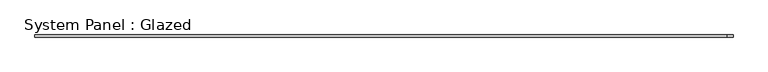
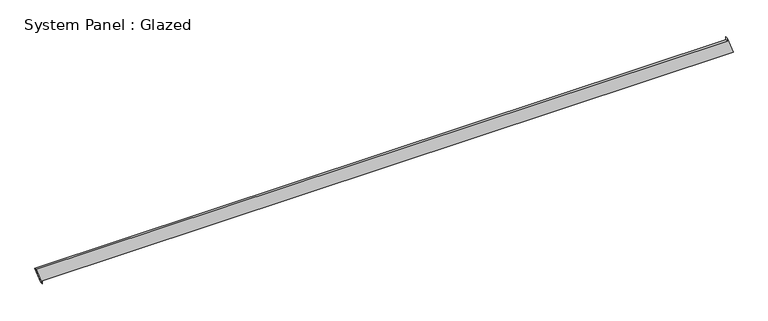
"""IFC4 building model written with IfcOpenShell, lengths in millimetres: plate geometry, System Panel : Glazed."""

from ifc_helpers import new_model, si_unit, frame, origin, place, context, project, spatial, polyline, outline, extrude, source, transform, mapped, element, save


def system_panel_glazed_d03e2e0c(model_context):
    return source(origin(), model_context, "Body", "SweptSolid", [
        extrude(outline(polyline([(0.0, -3959.0543609), (35.3553391, -3959.0543609), (35.3553391, 4027.7767133), (234.8330521, 3959.2965957), (199.477713, 3959.2970385), (199.3776864, -4027.7767133), (0.0, -3959.0543609)])), frame((0.0, -49.5, 0.0), z_axis=(0.0, 1.0, 0.0), x_axis=(0.0, 0.0, 1.0)), (0.0, 0.0, 1.0), 25.0),
    ])


if __name__ == "__main__":
    model = new_model("IFC4")
    model_context = context("Model", 3, world=origin())
    ifc_project = project(units=[si_unit("LENGTHUNIT", "METRE", prefix="MILLI")], contexts=[model_context])
    site = spatial("IfcSite", under=ifc_project)
    building = spatial("IfcBuilding", under=site)
    placement = place(None, origin())
    system_panel_glazed_shape = system_panel_glazed_d03e2e0c(model_context)
    element("IfcPlate", 1, ObjectType="System Panel : Glazed", at=placement, inside=building, context=model_context, shape_type="MappedRepresentation", body=[
        mapped(system_panel_glazed_shape, transform((0.0, 0.0, 0.0), x_axis=(1.0, 0.0, 0.0), y_axis=(0.0, 1.0, 0.0), z_axis=(0.0, 0.0, 1.0))),
    ])
    save(model, "model.ifc")

# Revit data of these elements
# Element 1 (IfcPlate, "System Panel : Glazed")
#   Materials on its faces: "Glass"
# Materials
#   "Glass": class "Glass", colour RGB 218 227 224, transparency 0.85, Description = "Soda Lime Glass", Cost = 0
